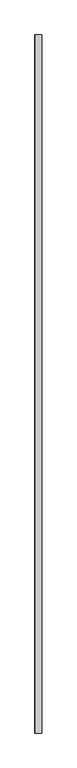
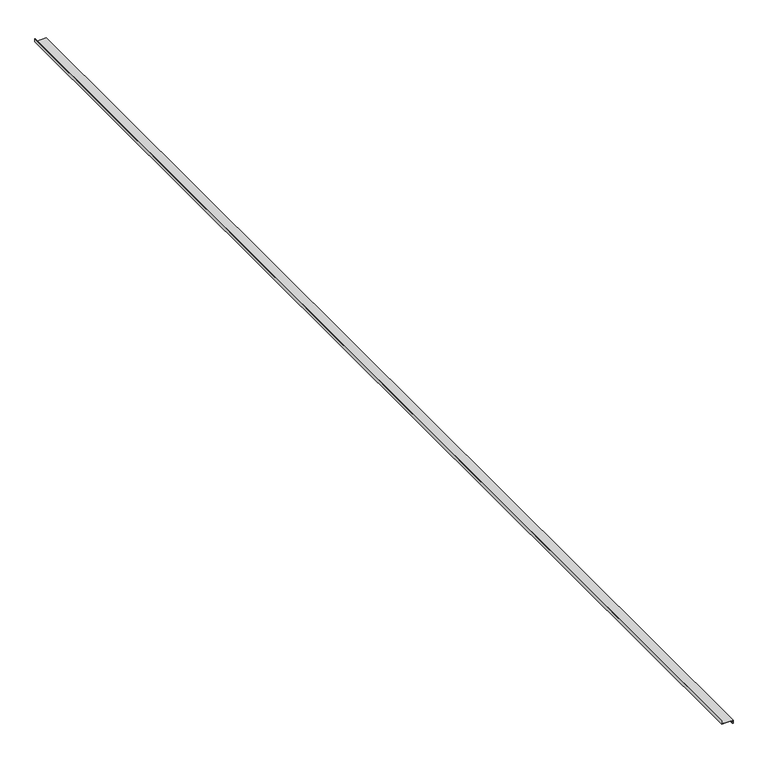
"""IFC4 building model written with IfcOpenShell, lengths in millimetres: proxy geometry, Generic Models 3:Generic Models 2:312240:Generic Models 2:312240 : Generic Models 3:Generic Models 2:312240:5 : Generic Models 3:Generic Models 2:312240:Generic Models 2:312240 : Generic Models 3:Generic Models 2:312240:300533."""

from ifc_helpers import new_model, si_unit, frame, origin, place, context, project, spatial, polyline, outline, extrude, source, transform, mapped, element, save


def generic_models_eeb2ffb5(model_context):
    return source(origin(), model_context, "Body", "SweptSolid", [
        extrude(outline(polyline([(-73.025, 667661.4718997), (-73.025, 667666.2343997), (-50.8, 667666.2343997), (-50.8, 667590.4166374), (-29.6633843, 667590.4166374), (-29.6633843, 667589.6228874), (-51.59375, 667589.6228874), (-51.59375, 667665.4406497), (-72.23125, 667665.4406497), (-72.23125, 667662.2656497), (-63.5, 667662.2656497), (-63.5, 667661.4718997), (-73.025, 667661.4718997)])), frame((0.0, -568253.9540363, 0.0), z_axis=(0.0, 1.0, 0.0), x_axis=(0.0, 0.0, 1.0)), (0.0, 0.0, 1.0), 7912.7376522),
    ])


if __name__ == "__main__":
    model = new_model("IFC4")
    model_context = context("Model", 3, world=origin())
    ifc_project = project(units=[si_unit("LENGTHUNIT", "METRE", prefix="MILLI")], contexts=[model_context])
    site = spatial("IfcSite", under=ifc_project)
    building = spatial("IfcBuilding", under=site)
    placement = place(None, origin())
    generic_models_shape = generic_models_eeb2ffb5(model_context)
    element("IfcBuildingElementProxy", 1, Name="Generic Models 3:Generic Models 2:312240:Generic Models 2:312240 : Generic Models 3:Generic Models 2:312240:5 : Generic Models 3:Generic Models 2:312240:Generic Models 2:312240 : Generic Models 3:Generic Models 2:312240:300533", ObjectType="Generic Models 3:Generic Models 2:312240:Generic Models 2:312240 : Generic Models 3:Generic Models 2:312240:5 : Generic Models 3:Generic Models 2:312240:Generic Models 2:312240 : Generic Models 3:Generic Models 2:312240:300533", at=placement, inside=building, context=model_context, shape_type="MappedRepresentation", body=[
        mapped(generic_models_shape, transform((0.0, 0.0, 0.0), x_axis=(1.0, 0.0, 0.0), y_axis=(0.0, 1.0, 0.0), z_axis=(0.0, 0.0, 1.0))),
    ])
    save(model, "model.ifc")

# Revit data of these elements
# Type "Generic Models 3:Generic Models 2:312240:Generic Models 2:312240 : Generic Models 3:Generic Models 2:312240:5 : Generic Models 3:Generic Models 2:312240:Generic Models 2:312240 : Generic Models 3:Generic Models 2:312240:300533"
#   NameOverride = "Generic Models 3:Generic Models 2:312240:Generic Models 2:312240 : Generic Models 3:Generic Models 2:312240:300533"
#   ObjectTypeOverride = "Generic Models 2:312240 : Generic Models 3:Generic Models 2:312240"
#   Reference = "Generic Models 2"
#   Tag = "300533"
# Element 1 (IfcBuildingElementProxy, "Generic Models 3:Generic Models 2:312240:Generic Models 2:312240 : Generic Models 3:Generic Models 2:312240:5 : Generic Models 3:Generic Models 2:312240:Generic Models 2:312240 : Generic Models 3:Generic Models 2:312240:300533")
#   Materials on its faces: "BRAKE METAL FLASHING WITH BACK & END DAMS"
# Materials
#   "BRAKE METAL FLASHING WITH BACK & END DAMS": class "Unassigned", colour RGB 182 182 182, transparency 0, Cost = 0
